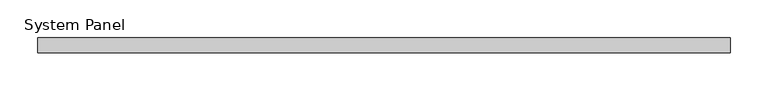
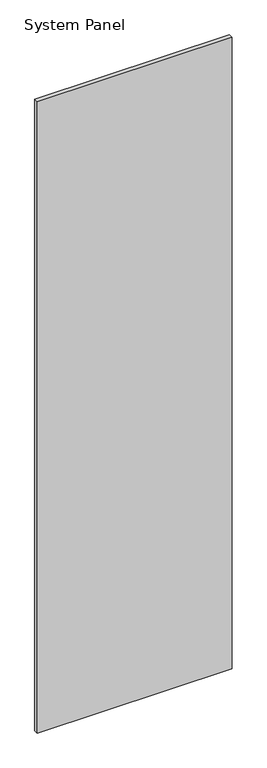
"""IFC4 building model written with IfcOpenShell, lengths in millimetres: plate geometry, System Panel : WWm-Glass-20mm-10mmOffset."""

from ifc_helpers import new_model, si_unit, origin, origin_with_axes, place, context, project, spatial, polyline, outline, extrude, source, transform, mapped, element, save


def system_panel_d54bef9b(model_context):
    return source(origin(), model_context, "Body", "SweptSolid", [
        extrude(outline(polyline([(460.0, 0.0), (-460.0, 0.0), (-460.0, 20.0), (460.0, 20.0), (460.0, 0.0)])), origin_with_axes(), (0.0, 0.0, 1.0), 3150.0),
    ])


if __name__ == "__main__":
    model = new_model("IFC4")
    model_context = context("Model", 3, world=origin())
    ifc_project = project(units=[si_unit("LENGTHUNIT", "METRE", prefix="MILLI")], contexts=[model_context])
    site = spatial("IfcSite", under=ifc_project)
    building = spatial("IfcBuilding", under=site)
    placement = place(None, origin())
    system_panel_shape = system_panel_d54bef9b(model_context)
    element("IfcPlate", 1, ObjectType="System Panel : WWm-Glass-20mm-10mmOffset", at=placement, inside=building, context=model_context, shape_type="MappedRepresentation", body=[
        mapped(system_panel_shape, transform((0.0, 0.0, 0.0), x_axis=(1.0, 0.0, 0.0), y_axis=(0.0, 1.0, 0.0), z_axis=(0.0, 0.0, 1.0))),
    ])
    save(model, "model.ifc")

# Revit data of these elements
# Type "System Panel : WWm-Glass-20mm-10mmOffset"
#   Finish = ""
# Element 1 (IfcPlate, "System Panel : WWm-Glass-20mm-10mmOffset")
#   Materials on its faces: "WW-EC-GL-Storefront"
# Materials
#   "WW-EC-GL-Storefront": class "Glass", colour RGB 236 240 239, transparency 0.85, Description = "Storefront Glass", Cost = 0
